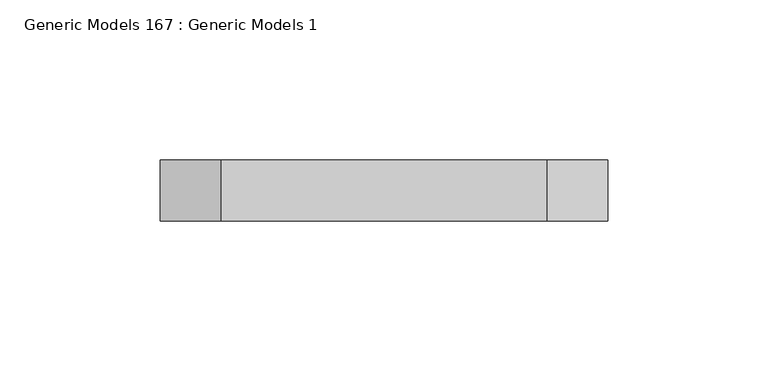
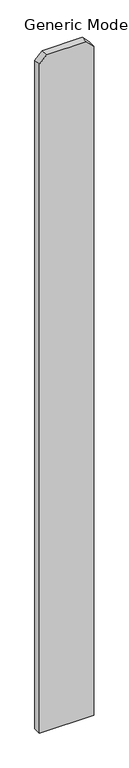
"""IFC4 building model written with IfcOpenShell, lengths in millimetres: proxy geometry, Generic Models 167 : Generic Models 1."""

import ifcopenshell
import ifcopenshell.guid

model = None  # the IFC model being written
_history = None  # IfcOwnerHistory: only IFC2X3 demands one
_inside = {}  # id of a spatial element -> (the spatial element, [elements in it])
_under = {}  # id of a project, library or spatial element -> (it, [spatial elements below it])
_declared = {}  # id of a project -> (the project, [libraries it declares])
_typed = {}  # id of a type object -> (the type object, [elements of that type])
_made_of = {}  # id of a material, layer set ... -> (it, [elements and type objects made of it])


def new_model(schema):
    """Start an empty IFC model of exactly this schema.

    Asked for "IFC4X3", IfcOpenShell would pick the latest addendum, in which some entities
    have other attributes; the version numbers below select the first issue.
    IFC2X3 requires an IfcOwnerHistory on every rooted entity: one is made here for all.
    """
    global model, _history
    if schema == "IFC4X3":
        model = ifcopenshell.file(schema_version=(4, 3, 0, 0))
    else:
        model = ifcopenshell.file(schema=schema)
    _inside.clear()
    _under.clear()
    _declared.clear()
    _typed.clear()
    _made_of.clear()
    _history = None
    if model.schema == "IFC2X3":
        org = make("IfcOrganization", Name="unknown")
        user = make(
            "IfcPersonAndOrganization",
            ThePerson=make("IfcPerson", FamilyName="unknown"),
            TheOrganization=org,
        )
        app = make(
            "IfcApplication",
            ApplicationDeveloper=org,
            Version="unknown",
            ApplicationFullName="unknown",
            ApplicationIdentifier="unknown",
        )
        _history = make(
            "IfcOwnerHistory",
            OwningUser=user,
            OwningApplication=app,
            ChangeAction="ADDED",
            CreationDate=0,
        )
    return model


def make(cls, **values):
    """One entity of the class cls with the attributes given. An attribute that is None is left unset."""
    return model.create_entity(
        cls, **{name: value for name, value in values.items() if value is not None}
    )


def rooted(cls, **values):
    """An entity with a GlobalId (a new one), such as an element, a storey or a relation."""
    return make(cls, GlobalId=ifcopenshell.guid.new(), OwnerHistory=_history, **values)


def si_unit(unit_type, name, prefix=None):
    """IfcSIUnit, for example si_unit("LENGTHUNIT", "METRE", prefix="MILLI")."""
    return make("IfcSIUnit", UnitType=unit_type, Prefix=prefix, Name=name)


def assignment(units):
    """IfcUnitAssignment: the units of a project."""
    return None if units is None else make("IfcUnitAssignment", Units=units)


def point(xyz):
    """IfcCartesianPoint."""
    return None if xyz is None else make("IfcCartesianPoint", Coordinates=xyz)


def direction(xyz):
    """IfcDirection."""
    return None if xyz is None else make("IfcDirection", DirectionRatios=xyz)


def frame(location, z_axis=None, x_axis=None):
    """IfcAxis2Placement3D, a coordinate frame: its origin and axes. An axis left out is left unset."""
    return make(
        "IfcAxis2Placement3D",
        Location=point(location),
        Axis=direction(z_axis),
        RefDirection=direction(x_axis),
    )


def origin():
    """The frame at (0, 0, 0) with its axes left unset."""
    return frame((0.0, 0.0, 0.0))


def place(relative_to, where):
    """IfcLocalPlacement: puts the frame where relative to a parent placement (None: the world)."""
    return make(
        "IfcLocalPlacement", PlacementRelTo=relative_to, RelativePlacement=where
    )


def context(
    kind, dimensions, precision=None, world=None, true_north=None, identifier=None
):
    """IfcGeometricRepresentationContext, for example the 3D "Model" context."""
    return make(
        "IfcGeometricRepresentationContext",
        ContextIdentifier=identifier,
        ContextType=kind,
        CoordinateSpaceDimension=dimensions,
        Precision=precision,
        WorldCoordinateSystem=world,
        TrueNorth=true_north,
    )


def project(units=None, contexts=None):
    """IfcProject with its units and contexts."""
    return rooted(
        "IfcProject",
        Name="project",
        RepresentationContexts=contexts,
        UnitsInContext=assignment(units),
    )


def spatial(cls, under=None, at=None, **own):
    """A site, building, storey or space (cls), placed at a placement, below another one or the project."""
    s = rooted(cls, ObjectPlacement=at, **own)
    if under is not None:
        _under.setdefault(under.id(), (under, []))[1].append(s)
    return s


def polyline(points):
    """IfcPolyline through the points."""
    return make("IfcPolyline", Points=[point(p) for p in points])


def outline(outer, holes=None, kind="AREA"):
    """IfcArbitraryClosedProfileDef: a profile drawn as a closed curve; with holes, ...WithVoids."""
    if holes is None:
        return make("IfcArbitraryClosedProfileDef", ProfileType=kind, OuterCurve=outer)
    return make(
        "IfcArbitraryProfileDefWithVoids",
        ProfileType=kind,
        OuterCurve=outer,
        InnerCurves=holes,
    )


def extrude(swept, where, along, depth):
    """IfcExtrudedAreaSolid: the profile swept, set in the frame where, extruded along a direction by depth."""
    return make(
        "IfcExtrudedAreaSolid",
        SweptArea=swept,
        Position=where,
        ExtrudedDirection=direction(along),
        Depth=depth,
    )


def shape(context_of_items, identifier, shape_type, items):
    """IfcShapeRepresentation: the items that make up one representation, for example the "Body"."""
    return make(
        "IfcShapeRepresentation",
        ContextOfItems=context_of_items,
        RepresentationIdentifier=identifier,
        RepresentationType=shape_type,
        Items=items,
    )


def source(mapping_origin, context_of_items, identifier, shape_type, items):
    """IfcRepresentationMap: a shape defined once, which mapped items show again and again."""
    return make(
        "IfcRepresentationMap",
        MappingOrigin=mapping_origin,
        MappedRepresentation=shape(context_of_items, identifier, shape_type, items),
    )


def transform(
    local_origin,
    x_axis=None,
    y_axis=None,
    z_axis=None,
    scale=None,
    scale2=None,
    scale3=None,
    uniform=True,
):
    """IfcCartesianTransformationOperator3D, or its non-uniform kind. x_axis, y_axis, z_axis: its Axis1, 2, 3."""
    if uniform:
        return make(
            "IfcCartesianTransformationOperator3D",
            Axis1=direction(x_axis),
            Axis2=direction(y_axis),
            LocalOrigin=point(local_origin),
            Scale=scale,
            Axis3=direction(z_axis),
        )
    return make(
        "IfcCartesianTransformationOperator3DnonUniform",
        Axis1=direction(x_axis),
        Axis2=direction(y_axis),
        LocalOrigin=point(local_origin),
        Scale=scale,
        Axis3=direction(z_axis),
        Scale2=scale2,
        Scale3=scale3,
    )


def mapped(mapping_source, mapping_target):
    """IfcMappedItem: shows the shape of a source again, moved by a transform."""
    return make(
        "IfcMappedItem", MappingSource=mapping_source, MappingTarget=mapping_target
    )


def made_of(thing, what):
    """Note that an element or type object is made of a material, layer set ...; save() writes the relation."""
    if what is not None:
        _made_of.setdefault(what.id(), (what, []))[1].append(thing)
    return thing


def element(
    cls,
    number,
    at=None,
    inside=None,
    cuts=None,
    type_object=None,
    material=None,
    context=None,
    identifier="Body",
    shape_type=None,
    held_by="IfcProductDefinitionShape",
    body=None,
    shapes=None,
    **own,
):
    """One element of the class cls, such as IfcWall. Its Tag is "e" and its number.

    at: its placement. inside: the storey or other place that contains it. cuts: it is an
    opening in that element (IfcRelVoidsElement). A single representation is given by context,
    identifier, shape_type and body (its items); several are given by shapes. held_by: the class
    of the entity that holds the representations. save() writes the other relations.
    """
    e = rooted(cls, Tag="e%d" % number, ObjectPlacement=at, **own)
    if body is not None:
        shapes = [shape(context, identifier, shape_type, body)]
    if shapes is not None:
        e.Representation = make(held_by, Representations=shapes)
    if inside is not None:
        _inside.setdefault(inside.id(), (inside, []))[1].append(e)
    if cuts is not None:
        rooted(
            "IfcRelVoidsElement", RelatingBuildingElement=cuts, RelatedOpeningElement=e
        )
    if type_object is not None:
        _typed.setdefault(type_object.id(), (type_object, []))[1].append(e)
    return made_of(e, material)


def aggregate(whole, parts):
    """IfcRelAggregates: a whole, such as a stair, and the parts it consists of."""
    return rooted("IfcRelAggregates", RelatingObject=whole, RelatedObjects=parts)


def save(model, path):
    """Write the relations noted so far, then the file.

    IfcRelAggregates (storeys below a building ...), IfcRelContainedInSpatialStructure (elements
    in a storey), IfcRelDefinesByType, IfcRelAssociatesMaterial and IfcRelDeclares: one each for
    every whole, place, type object, material and project.
    """
    for whole, parts in _under.values():
        aggregate(whole, parts)
    for where, things in _inside.values():
        rooted(
            "IfcRelContainedInSpatialStructure",
            RelatedElements=things,
            RelatingStructure=where,
        )
    for kind, things in _typed.values():
        rooted("IfcRelDefinesByType", RelatedObjects=things, RelatingType=kind)
    for what, things in _made_of.values():
        rooted("IfcRelAssociatesMaterial", RelatedObjects=things, RelatingMaterial=what)
    for by, libraries in _declared.values():
        rooted("IfcRelDeclares", RelatingContext=by, RelatedDefinitions=libraries)
    model.write(path)


def generic_models_167_generic_models_1_3792af48(model_context):
    return source(origin(), model_context, "Body", "SweptSolid", [
        extrude(outline(polyline([(76.2, 55446.6125), (1885.95, 55446.6125), (1905.0, 55427.5625), (1905.0, 55325.9625), (1885.95, 55306.9125), (76.2, 55306.9125), (76.2, 55446.6125)])), frame((0.0, 547.6875, 0.0), z_axis=(0.0, 1.0, 0.0), x_axis=(0.0, 0.0, 1.0)), (0.0, 0.0, 1.0), 19.05),
    ])


if __name__ == "__main__":
    model = new_model("IFC4")
    model_context = context("Model", 3, world=origin())
    ifc_project = project(units=[si_unit("LENGTHUNIT", "METRE", prefix="MILLI")], contexts=[model_context])
    site = spatial("IfcSite", under=ifc_project)
    building = spatial("IfcBuilding", under=site)
    placement = place(None, origin())
    generic_models_167_generic_models_1_shape = generic_models_167_generic_models_1_3792af48(model_context)
    element("IfcBuildingElementProxy", 1, Name="Generic Models 167 : Generic Models 1", ObjectType="Generic Models 167 : Generic Models 1", at=placement, inside=building, context=model_context, shape_type="MappedRepresentation", body=[
        mapped(generic_models_167_generic_models_1_shape, transform((0.0, 0.0, 0.0), x_axis=(1.0, 0.0, 0.0), y_axis=(0.0, 1.0, 0.0), z_axis=(0.0, 0.0, 1.0))),
    ])
    save(model, "model.ifc")

# Revit data of these elements
# Element 1 (IfcBuildingElementProxy, "Generic Models 167 : Generic Models 1")
#   Materials on its faces: "VERTICAL 1X6 CEDAR PLANKS W/ CLEAR WOOD SEALER"
# Materials
#   "VERTICAL 1X6 CEDAR PLANKS W/ CLEAR WOOD SEALER": class "Wood", colour RGB 234 198 147, transparency 0, Description = "Pinus Echinata", Cost = 0
